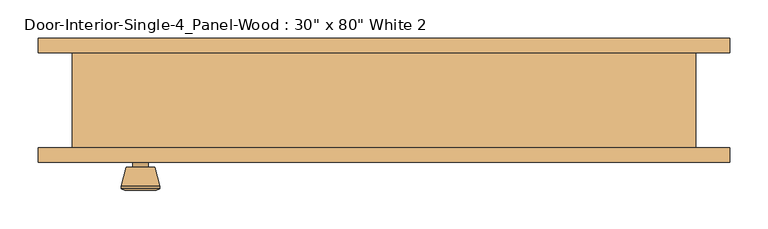
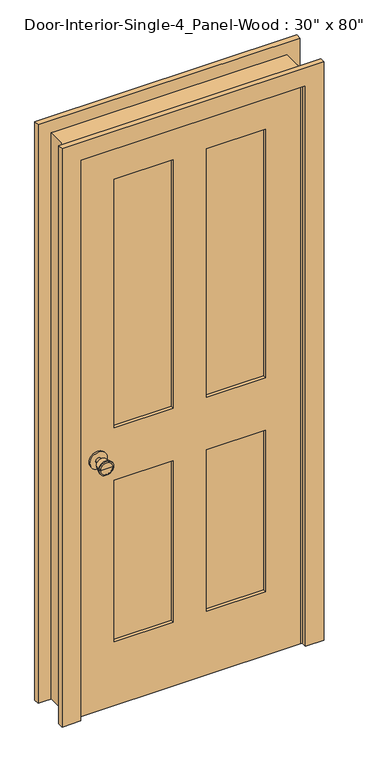
"""IFC4 building model written with IfcOpenShell, lengths in millimetres: door geometry."""

from ifc_helpers import new_model, si_unit, point, frame, frame_2d, origin, place, context, project, spatial, polyline, circle_curve, trimmed, segment, composite_curve, outline, extrude, faceted_brep, source, transform, mapped, element, save
from ifc_brep_helpers import plane_surface, cylinder_surface, revolved_surface, advanced_brep


def door_60a06af2(model_context):
    return source(origin(), model_context, "Body", "SolidModel", [
        advanced_brep(
        [(-317.5, -17.8125, 914.4), (-327.5, -17.8125, 914.4), (-307.5, -17.8125, 914.4), (-297.0241324, 31.1875, 914.4), (-337.9758676, 31.1875, 914.4), (-317.5, 31.1875, 914.4), (-292.5, 29.3596319, 914.4), (-342.5, 29.3596319, 914.4), (-292.5, 25.8959537, 914.4), (-342.5, 25.8959537, 914.4), (-298.863764, 1.1875, 914.4), (-336.136236, 1.1875, 914.4), (-307.5, 1.1875, 914.4), (-327.5, 1.1875, 914.4)],
        [
            (0, 1),
            (1, 2, circle_curve(frame((-317.5, -17.8125, 914.4), z_axis=(0.0, -1.0, 0.0), x_axis=(-1.0, 0.0, 0.0)), 10.0)),
            (2, 0),
            (2, 1, circle_curve(frame((-317.5, -17.8125, 914.4), z_axis=(0.0, -1.0, 0.0), x_axis=(-1.0, 0.0, 0.0)), 10.0)),
            (3, 4, circle_curve(frame((-317.5, 31.1875, 914.4), z_axis=(0.0, 1.0, 0.0), x_axis=(-1.0, 0.0, 0.0)), 20.4758676)),
            (4, 5),
            (5, 3),
            (4, 3, circle_curve(frame((-317.5, 31.1875, 914.4), z_axis=(0.0, 1.0, 0.0), x_axis=(-1.0, 0.0, 0.0)), 20.4758676)),
            (6, 7, circle_curve(frame((-317.5, 29.3596319, 914.4), z_axis=(0.0, 1.0, 0.0), x_axis=(-1.0, 0.0, 0.0)), 25.0)),
            (7, 4),
            (3, 6),
            (7, 6, circle_curve(frame((-317.5, 29.3596319, 914.4), z_axis=(0.0, 1.0, 0.0), x_axis=(-1.0, 0.0, 0.0)), 25.0)),
            (8, 9, circle_curve(frame((-317.5, 25.8959537, 914.4), z_axis=(0.0, 1.0, 0.0), x_axis=(-1.0, 0.0, 0.0)), 25.0)),
            (9, 7),
            (6, 8),
            (9, 8, circle_curve(frame((-317.5, 25.8959537, 914.4), z_axis=(0.0, 1.0, 0.0), x_axis=(-1.0, 0.0, 0.0)), 25.0)),
            (10, 11, circle_curve(frame((-317.5, 1.1875, 914.4), z_axis=(0.0, 1.0, 0.0), x_axis=(-1.0, 0.0, 0.0)), 18.636236)),
            (11, 9),
            (8, 10),
            (11, 10, circle_curve(frame((-317.5, 1.1875, 914.4), z_axis=(0.0, 1.0, 0.0), x_axis=(-1.0, 0.0, 0.0)), 18.636236)),
            (12, 13, circle_curve(frame((-317.5, 1.1875, 914.4), z_axis=(0.0, 1.0, 0.0), x_axis=(-1.0, 0.0, 0.0)), 10.0)),
            (13, 11),
            (10, 12),
            (13, 12, circle_curve(frame((-317.5, 1.1875, 914.4), z_axis=(0.0, 1.0, 0.0), x_axis=(-1.0, 0.0, 0.0)), 10.0)),
            (1, 13),
            (12, 2),
        ],
        [
            plane_surface(frame((-317.5, -17.8125, 914.4), z_axis=(0.0, -1.0, 0.0), x_axis=(-1.0, 0.0, 0.0))),
            plane_surface(frame((-317.5, 31.1875, 914.4), z_axis=(0.0, 1.0, 0.0), x_axis=(-1.0, 0.0, 0.0))),
            revolved_surface(polyline([(-337.9758676, 31.1875, 914.4), (-342.5, 29.3596319, 914.4)]), (-317.5, -17.8125, 914.4), (0.0, -1.0, 0.0)),
            cylinder_surface(frame((-317.5, -17.8125, 914.4), z_axis=(0.0, -1.0, 0.0), x_axis=(-1.0, 0.0, 0.0)), 25.0),
            revolved_surface(polyline([(-342.5, 25.8959537, 914.4), (-336.136236, 1.1875, 914.4)]), (-317.5, -17.8125, 914.4), (0.0, -1.0, 0.0)),
            plane_surface(frame((-317.5, 1.1875, 914.4), z_axis=(0.0, -1.0, 0.0), x_axis=(-1.0, 0.0, 0.0))),
            cylinder_surface(frame((-317.5, -17.8125, 914.4), z_axis=(0.0, -1.0, 0.0), x_axis=(-1.0, 0.0, 0.0)), 10.0),
        ],
        [
            (0, [[1, 2, 3]]),
            (0, [[-3, 4, -1]]),
            (1, [[5, 6, 7]]),
            (1, [[8, -7, -6]]),
            (2, [[9, 10, -5, 11]]),
            (2, [[12, -11, -8, -10]]),
            (3, [[13, 14, -9, 15]]),
            (3, [[16, -15, -12, -14]]),
            (4, [[17, 18, -13, 19]]),
            (4, [[20, -19, -16, -18]]),
            (5, [[21, 22, -17, 23]]),
            (5, [[24, -23, -20, -22]]),
            (6, [[-2, 25, -21, 26]]),
            (6, [[-4, -26, -24, -25]]),
        ],
    ),
        extrude(outline(composite_curve([segment(trimmed(circle_curve(frame_2d((914.4, -317.5)), 30.0), [point((914.4, -347.5))], [point((914.4, -287.5))], False, "CARTESIAN"), True, "CONTINUOUS"), segment(trimmed(circle_curve(frame_2d((914.4, -317.5)), 30.0), [point((914.4, -287.5))], [point((914.4, -347.5))], False, "CARTESIAN"), True, "CONTINUOUS")], self_intersect=False)), frame((0.0, -23.8125, 0.0), z_axis=(0.0, 1.0, 0.0), x_axis=(0.0, 0.0, 1.0)), (0.0, 0.0, 1.0), 6.0),
        advanced_brep(
        [(-317.5, -64.7375, 914.4), (-307.5, -64.7375, 914.4), (-327.5, -64.7375, 914.4), (-297.0241324, -113.7375, 914.4), (-317.5, -113.7375, 914.4), (-337.9758676, -113.7375, 914.4), (-292.5, -111.9096319, 914.4), (-342.5, -111.9096319, 914.4), (-292.5, -108.4459537, 914.4), (-342.5, -108.4459537, 914.4), (-298.863764, -83.7375, 914.4), (-336.136236, -83.7375, 914.4), (-307.5, -83.7375, 914.4), (-327.5, -83.7375, 914.4)],
        [
            (0, 1),
            (1, 2, circle_curve(frame((-317.5, -64.7375, 914.4), z_axis=(0.0, 1.0, 0.0), x_axis=(-1.0, 0.0, 0.0)), 10.0)),
            (2, 0),
            (2, 1, circle_curve(frame((-317.5, -64.7375, 914.4), z_axis=(0.0, 1.0, 0.0), x_axis=(-1.0, 0.0, 0.0)), 10.0)),
            (3, 4),
            (4, 5),
            (5, 3, circle_curve(frame((-317.5, -113.7375, 914.4), z_axis=(0.0, -1.0, 0.0), x_axis=(-1.0, 0.0, 0.0)), 20.4758676)),
            (3, 5, circle_curve(frame((-317.5, -113.7375, 914.4), z_axis=(0.0, -1.0, 0.0), x_axis=(-1.0, 0.0, 0.0)), 20.4758676)),
            (6, 3),
            (5, 7),
            (7, 6, circle_curve(frame((-317.5, -111.9096319, 914.4), z_axis=(0.0, -1.0, 0.0), x_axis=(-1.0, 0.0, 0.0)), 25.0)),
            (6, 7, circle_curve(frame((-317.5, -111.9096319, 914.4), z_axis=(0.0, -1.0, 0.0), x_axis=(-1.0, 0.0, 0.0)), 25.0)),
            (8, 6),
            (7, 9),
            (9, 8, circle_curve(frame((-317.5, -108.4459537, 914.4), z_axis=(0.0, -1.0, 0.0), x_axis=(-1.0, 0.0, 0.0)), 25.0)),
            (8, 9, circle_curve(frame((-317.5, -108.4459537, 914.4), z_axis=(0.0, -1.0, 0.0), x_axis=(-1.0, 0.0, 0.0)), 25.0)),
            (10, 8),
            (9, 11),
            (11, 10, circle_curve(frame((-317.5, -83.7375, 914.4), z_axis=(0.0, -1.0, 0.0), x_axis=(-1.0, 0.0, 0.0)), 18.636236)),
            (10, 11, circle_curve(frame((-317.5, -83.7375, 914.4), z_axis=(0.0, -1.0, 0.0), x_axis=(-1.0, 0.0, 0.0)), 18.636236)),
            (12, 10),
            (11, 13),
            (13, 12, circle_curve(frame((-317.5, -83.7375, 914.4), z_axis=(0.0, -1.0, 0.0), x_axis=(-1.0, 0.0, 0.0)), 10.0)),
            (12, 13, circle_curve(frame((-317.5, -83.7375, 914.4), z_axis=(0.0, -1.0, 0.0), x_axis=(-1.0, 0.0, 0.0)), 10.0)),
            (1, 12),
            (13, 2),
        ],
        [
            plane_surface(frame((-317.5, -64.7375, 914.4), z_axis=(0.0, 1.0, 0.0), x_axis=(-1.0, 0.0, 0.0))),
            plane_surface(frame((-317.5, -113.7375, 914.4), z_axis=(0.0, -1.0, 0.0), x_axis=(-1.0, 0.0, 0.0))),
            revolved_surface(polyline([(-337.9758676, -113.7375, 914.4), (-342.5, -111.9096319, 914.4)]), (-317.5, -64.7375, 914.4), (0.0, 1.0, 0.0)),
            cylinder_surface(frame((-317.5, -64.7375, 914.4), z_axis=(0.0, 1.0, 0.0), x_axis=(-1.0, 0.0, 0.0)), 25.0),
            revolved_surface(polyline([(-342.5, -108.4459537, 914.4), (-336.136236, -83.7375, 914.4)]), (-317.5, -64.7375, 914.4), (0.0, 1.0, 0.0)),
            plane_surface(frame((-317.5, -83.7375, 914.4), z_axis=(0.0, 1.0, 0.0), x_axis=(-1.0, 0.0, 0.0))),
            cylinder_surface(frame((-317.5, -64.7375, 914.4), z_axis=(0.0, 1.0, 0.0), x_axis=(-1.0, 0.0, 0.0)), 10.0),
        ],
        [
            (0, [[1, 2, 3]]),
            (0, [[-3, 4, -1]]),
            (1, [[5, 6, 7]]),
            (1, [[-6, -5, 8]]),
            (2, [[9, -7, 10, 11]]),
            (2, [[-10, -8, -9, 12]]),
            (3, [[13, -11, 14, 15]]),
            (3, [[-14, -12, -13, 16]]),
            (4, [[17, -15, 18, 19]]),
            (4, [[-18, -16, -17, 20]]),
            (5, [[21, -19, 22, 23]]),
            (5, [[-22, -20, -21, 24]]),
            (6, [[25, -23, 26, -2]]),
            (6, [[-26, -24, -25, -4]]),
        ],
    ),
        extrude(outline(composite_curve([segment(trimmed(circle_curve(frame_2d((914.4, -317.5)), 30.0), [point((914.4, -347.5))], [point((914.4, -287.5))], False, "CARTESIAN"), True, "CONTINUOUS"), segment(trimmed(circle_curve(frame_2d((914.4, -317.5)), 30.0), [point((914.4, -287.5))], [point((914.4, -347.5))], False, "CARTESIAN"), True, "CONTINUOUS")], self_intersect=False)), frame((0.0, -64.7375, 0.0), z_axis=(0.0, 1.0, 0.0), x_axis=(0.0, 0.0, 1.0)), (0.0, 0.0, 1.0), 6.0),
        extrude(outline(polyline([(260.35, -35.4541667), (260.35, -47.0958333), (57.15, -47.0958333), (57.15, -35.4541667), (260.35, -35.4541667)])), frame((0.0, 0.0, 1009.65), z_axis=(0.0, 0.0, 1.0), x_axis=(1.0, 0.0, 0.0)), (0.0, 0.0, 1.0), 903.2875),
        extrude(outline(polyline([(-57.15, -35.4541667), (-57.15, -47.0958333), (-260.35, -47.0958333), (-260.35, -35.4541667), (-57.15, -35.4541667)])), frame((0.0, 0.0, 1009.65), z_axis=(0.0, 0.0, 1.0), x_axis=(1.0, 0.0, 0.0)), (0.0, 0.0, 1.0), 903.2875),
        extrude(outline(polyline([(260.35, -35.4541667), (260.35, -47.0958333), (57.15, -47.0958333), (57.15, -35.4541667), (260.35, -35.4541667)])), frame((0.0, 0.0, 231.775), z_axis=(0.0, 0.0, 1.0), x_axis=(1.0, 0.0, 0.0)), (0.0, 0.0, 1.0), 587.375),
        extrude(outline(polyline([(-57.15, -35.4541667), (-57.15, -47.0958333), (-260.35, -47.0958333), (-260.35, -35.4541667), (-57.15, -35.4541667)])), frame((0.0, 0.0, 231.775), z_axis=(0.0, 0.0, 1.0), x_axis=(1.0, 0.0, 0.0)), (0.0, 0.0, 1.0), 587.375),
        extrude(outline(polyline([(2032.0, -381.0), (0.0, -381.0), (0.0, 381.0), (2032.0, 381.0), (2032.0, -381.0)]), holes=[polyline([(1912.9375, 57.15), (1912.9375, 260.35), (1009.65, 260.35), (1009.65, 57.15), (1912.9375, 57.15)]), polyline([(1009.65, -57.15), (1009.65, -260.35), (1912.9375, -260.35), (1912.9375, -57.15), (1009.65, -57.15)]), polyline([(819.15, 57.15), (819.15, 260.35), (231.775, 260.35), (231.775, 57.15), (819.15, 57.15)]), polyline([(231.775, -57.15), (231.775, -260.35), (819.15, -260.35), (819.15, -57.15), (231.775, -57.15)])]), frame((0.0, -58.7375, 0.0), z_axis=(0.0, 1.0, 0.0), x_axis=(0.0, 0.0, 1.0)), (0.0, 0.0, 1.0), 34.925),
        faceted_brep([(406.4, -58.7375, 0.0), (381.0, -58.7375, 0.0), (381.0, -23.8125, 0.0), (368.3, -23.8125, 0.0), (368.3, 11.1125, 0.0), (381.0, 11.1125, 0.0), (381.0, 65.0875, 0.0), (406.4, 65.0875, 0.0), (406.4, 65.0875, 2057.4), (406.4, -58.7375, 2057.4), (381.0, 65.0875, 2032.0), (-381.0, 65.0875, 2032.0), (-381.0, 65.0875, 0.0), (-406.4, 65.0875, 0.0), (-406.4, 65.0875, 2057.4), (381.0, 11.1125, 2032.0), (368.3, 11.1125, 2019.3), (-368.3, 11.1125, 2019.3), (-368.3, 11.1125, 0.0), (-381.0, 11.1125, 0.0), (-381.0, 11.1125, 2032.0), (368.3, -23.8125, 2019.3), (381.0, -23.8125, 2032.0), (-381.0, -23.8125, 2032.0), (-381.0, -23.8125, 0.0), (-368.3, -23.8125, 0.0), (-368.3, -23.8125, 2019.3), (381.0, -58.7375, 2032.0), (-406.4, -58.7375, 2057.4), (-406.4, -58.7375, 0.0), (-381.0, -58.7375, 0.0), (-381.0, -58.7375, 2032.0)], [[[0, 1, 2, 3, 4, 5, 6, 7]], [[7, 8, 9, 0]], [[6, 10, 11, 12, 13, 14, 8, 7]], [[5, 15, 10, 6]], [[4, 16, 17, 18, 19, 20, 15, 5]], [[3, 21, 16, 4]], [[2, 22, 23, 24, 25, 26, 21, 3]], [[1, 27, 22, 2]], [[0, 9, 28, 29, 30, 31, 27, 1]], [[8, 14, 28, 9]], [[15, 20, 11, 10]], [[21, 26, 17, 16]], [[27, 31, 23, 22]], [[29, 13, 12, 19, 18, 25, 24, 30]], [[14, 13, 29, 28]], [[20, 19, 12, 11]], [[26, 25, 18, 17]], [[31, 30, 24, 23]]]),
        extrude(outline(polyline([(0.0, 450.85), (2101.85, 450.85), (2101.85, -450.85), (0.0, -450.85), (0.0, -387.35), (2038.35, -387.35), (2038.35, 387.35), (0.0, 387.35), (0.0, 450.85)])), frame((0.0, 65.0875, 0.0), z_axis=(0.0, 1.0, 0.0), x_axis=(0.0, 0.0, 1.0)), (0.0, 0.0, 1.0), 19.05),
        extrude(outline(polyline([(0.0, 450.85), (2101.85, 450.85), (2101.85, -450.85), (0.0, -450.85), (0.0, -387.35), (2038.35, -387.35), (2038.35, 387.35), (0.0, 387.35), (0.0, 450.85)])), frame((0.0, -77.7875, 0.0), z_axis=(0.0, 1.0, 0.0), x_axis=(0.0, 0.0, 1.0)), (0.0, 0.0, 1.0), 19.05),
    ])


if __name__ == "__main__":
    model = new_model("IFC4")
    model_context = context("Model", 3, world=origin())
    ifc_project = project(units=[si_unit("LENGTHUNIT", "METRE", prefix="MILLI")], contexts=[model_context])
    site = spatial("IfcSite", under=ifc_project)
    building = spatial("IfcBuilding", under=site)
    placement = place(None, origin())
    door_shape = door_60a06af2(model_context)
    element("IfcDoor", 1, ObjectType="Door-Interior-Single-4_Panel-Wood : 30\" x 80\" White 2", at=placement, inside=building, context=model_context, shape_type="MappedRepresentation", body=[
        mapped(door_shape, transform((0.0, 0.0, 0.0), x_axis=(1.0, 0.0, 0.0), y_axis=(0.0, 1.0, 0.0), z_axis=(0.0, 0.0, 1.0))),
    ])
    save(model, "model.ifc")

# Revit data of these elements
# Type "Door-Interior-Single-4_Panel-Wood : 30\" x 80\" White 2"
#   Type Mark = "71"
#   COBie.Type.CreatedBy = "doug.wood@us.ibm.com"
#   COBie.Type.CreatedOn = "2016-04-14T02:07:24"
#   COBie.Type.Name = "Doors_Door-Interior-Single-4_Panel-Wood_30\" x 80\" White 2_71"
#   COBie.Type.Category = "23-30 10 00 : Doors"
#   COBie.Type.Description = "Door-Interior-Single-4_Panel-Wood_30\" x 80\" White 2"
#   COBie.Type.Manufacturer = ""
#   COBie.Type.ModelNumber = ""
#   Assembly Code = "C1020300"
#   Analytic Construction = "Wooden"
#   COBie.Type.ReplacementCost = 0
#   Top Rail = 0' - 4 11/16"
#   Thickness = 0' - 1 3/8"
#   Thermal Resistance (R) = 0.455703 (m²·K)/W
#   Swing Angle [instance default] = 90.00°
#   Stiles = 0' - 4 3/4"
#   Rough Width = 2' - 8"
#   Rough Height = 6' - 9"
#   Mullion = 0' - 4 1/2"
#   Lock Rail = 0' - 7 1/2"
#   Height = 6' - 8"
#   Width = 2' - 6"
#   Heat Transfer Coefficient (U) = 2.19465 W/(m²·K)
#   Bottom Rail = 0' - 9 1/8"
#   COBie.Type = no
#   Trim Material = Trim - White
#   Panel Material = Door - Panel - White
#   Frame Material = Door - Panel - White
#   Door Handle Material = ARCAT - Metal - Brass, Polished
#   Visual Light Transmittance = 0
#   Solar Heat Gain Coefficient = 0
#   Wall Closure = (empty or 0)
#   Function = (empty or 0)
# Element 1 (IfcDoor, "Door-Interior-Single-4_Panel-Wood : 30\" x 80\" White 2")
#   Materials on its faces: "Door - Panel - White", "ARCAT - Metal - Brass, Polished", "Trim - White"
# Materials
#   "Trim - White": class "Wood", colour RGB 255 255 255, transparency 0, Cost = 0
#   "Door - Panel - White": class "Wood", colour RGB 255 255 255, transparency 0, Cost = 0
#   "ARCAT - Metal - Brass, Polished": class "Unassigned", colour RGB 246 240 166, transparency 0, Keynote = "05050", Model = "Generic", Manufacturer = "Generic", Description = "Steel, Chrome Plated"
